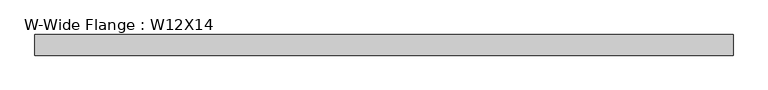
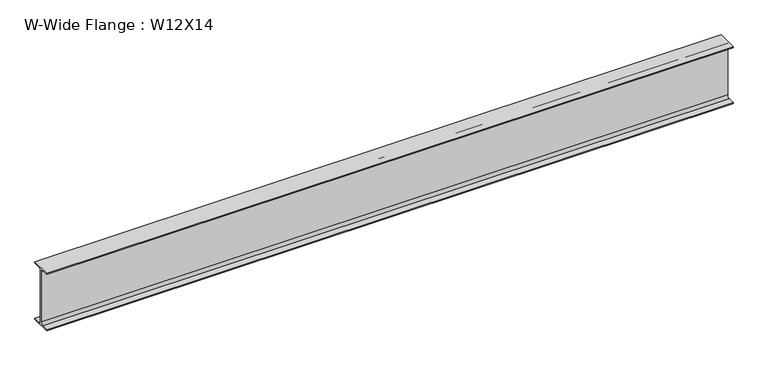
"""IFC4 building model written with IfcOpenShell, lengths in millimetres: beam geometry, W-Wide Flange : W12X14."""

from ifc_helpers import new_model, si_unit, point, frame, frame_2d, origin, place, context, project, spatial, polyline, circle_curve, trimmed, segment, composite_curve, outline, extrude, source, transform, mapped, element, save


def w_wide_flange_w12x14_19a1df3a(model_context):
    return source(origin(), model_context, "Body", "SweptSolid", [
        extrude(outline(composite_curve([segment(polyline([(50.419, -145.415), (50.419, -151.13), (-50.419, -151.13), (-50.419, -145.415), (-15.875, -145.415)]), True, "CONTINUOUS"), segment(trimmed(circle_curve(frame_2d((-15.875, -132.08)), 13.335), [point((-15.875, -145.415))], [point((-2.54, -132.08))], True, "CARTESIAN"), True, "CONTINUOUS"), segment(polyline([(-2.54, -132.08), (-2.54, 132.08)]), True, "CONTINUOUS"), segment(trimmed(circle_curve(frame_2d((-15.875, 132.08)), 13.335), [point((-2.54, 132.08))], [point((-15.875, 145.415))], True, "CARTESIAN"), True, "CONTINUOUS"), segment(polyline([(-15.875, 145.415), (-50.419, 145.415), (-50.419, 151.13), (50.419, 151.13), (50.419, 145.415), (15.875, 145.415)]), True, "CONTINUOUS"), segment(trimmed(circle_curve(frame_2d((15.875, 132.08)), 13.335), [point((15.875, 145.415))], [point((2.54, 132.08))], True, "CARTESIAN"), True, "CONTINUOUS"), segment(polyline([(2.54, 132.08), (2.54, -132.08)]), True, "CONTINUOUS"), segment(trimmed(circle_curve(frame_2d((15.875, -132.08)), 13.335), [point((2.54, -132.08))], [point((15.875, -145.415))], True, "CARTESIAN"), True, "CONTINUOUS"), segment(polyline([(15.875, -145.415), (50.419, -145.415)]), True, "CONTINUOUS")], self_intersect=False)), frame((-1739.9, 0.0, 0.0), z_axis=(1.0, 0.0, 0.0), x_axis=(0.0, 1.0, 0.0)), (0.0, 0.0, 1.0), 3416.173),
    ])


if __name__ == "__main__":
    model = new_model("IFC4")
    model_context = context("Model", 3, world=origin())
    ifc_project = project(units=[si_unit("LENGTHUNIT", "METRE", prefix="MILLI")], contexts=[model_context])
    site = spatial("IfcSite", under=ifc_project)
    building = spatial("IfcBuilding", under=site)
    placement = place(None, origin())
    w_wide_flange_w12x14_shape = w_wide_flange_w12x14_19a1df3a(model_context)
    element("IfcBeam", 1, ObjectType="W-Wide Flange : W12X14", at=placement, inside=building, context=model_context, shape_type="MappedRepresentation", body=[
        mapped(w_wide_flange_w12x14_shape, transform((0.0, 0.0, 0.0), x_axis=(1.0, 0.0, 0.0), y_axis=(0.0, 1.0, 0.0), z_axis=(0.0, 0.0, 1.0))),
    ])
    save(model, "model.ifc")

# Revit data of these elements
# Type "W-Wide Flange : W12X14"
#   Assembly Code = "B10"
#   W = 14
#   Length [instance default] = 5' - 0"
#   bf = 0' - 3.97"
#   d = 0' - 11.9"
#   k = 0' - 0 3/4"
#   k2 = 0' - 0.525"
#   tf = 0' - 0.225"
#   tw = 0' - 0.2"
#   A = 0.0288889 SF
#   Structural Material [instance default] = Steel ASTM A992
# Element 1 (IfcBeam, "W-Wide Flange : W12X14")
#   Materials on its faces: "Steel ASTM A992"
# Materials
#   "Steel ASTM A992": class "Metal", colour RGB 199 199 199, transparency 0, Description = "Structural steel 50ksi", Cost = 0
